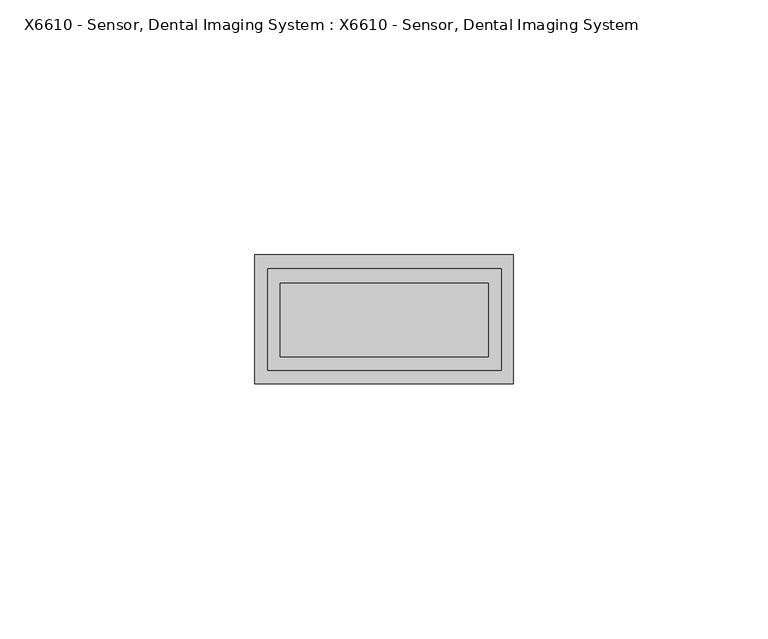
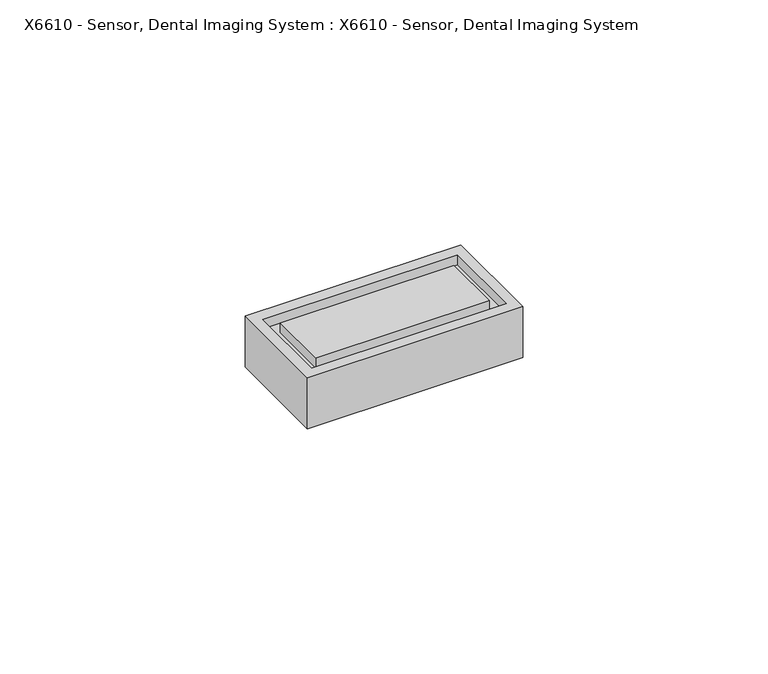
"""IFC4 building model written with IfcOpenShell, lengths in millimetres: proxy geometry, X6610 - Sensor, Dental Imaging System : X6610 - Sensor, Dental Imaging System."""

from ifc_helpers import new_model, si_unit, frame, origin, place, context, project, spatial, polyline, outline, extrude, faceted_brep, source, transform, mapped, element, save


def x6610_sensor_dental_imaging_system_x6610_sensor_dental_c57a1d08(model_context):
    return source(origin(), model_context, "Body", "SolidModel", [
        extrude(outline(polyline([(20.4811453, 7.060747), (20.4811453, -7.3741427), (-20.3347495, -7.3741427), (-20.3347495, 7.060747), (20.4811453, 7.060747)])), frame((0.0, 0.0, 10.2472794), z_axis=(0.0, 0.0, 1.0), x_axis=(1.0, 0.0, 0.0)), (0.0, 0.0, 1.0), 2.4527206),
        faceted_brep([(25.4, -12.7, 12.7), (-25.4, -12.7, 12.7), (-25.4, -12.7, 0.0), (25.4, -12.7, 0.0), (25.4, 12.7, 12.7), (25.4, 12.7, 0.0), (-25.4, 12.7, 0.0), (-25.4, 12.7, 12.7), (-22.8050147, 9.9039698, 12.7), (22.9818235, 9.9039698, 12.7), (22.9818235, -10.029614, 12.7), (-22.8050147, -10.029614, 12.7), (25.4, -5.9907412, 2.9524929), (25.4, -5.9907412, 7.2153756), (25.4, 6.0970829, 7.2153756), (25.4, 6.0970829, 2.9524929), (22.9818235, 9.9039698, 10.2472794), (-22.8050147, 9.9039698, 10.2472794), (-22.8050147, -10.029614, 10.2472794), (22.9818235, -10.029614, 10.2472794), (17.7337242, -5.9907412, 7.2153756), (17.7337242, -5.9907412, 2.9524929), (17.7337242, 6.0970829, 2.9524929), (17.7337242, 6.0970829, 7.2153756)], [[[0, 1, 2, 3]], [[4, 5, 6, 7]], [[1, 0, 4, 7], [8, 9, 10, 11]], [[2, 1, 7, 6]], [[3, 2, 6, 5]], [[0, 3, 5, 4], [12, 13, 14, 15]], [[16, 17, 18, 19]], [[17, 16, 9, 8]], [[18, 17, 8, 11]], [[19, 18, 11, 10]], [[16, 19, 10, 9]], [[20, 21, 22, 23]], [[21, 20, 13, 12]], [[22, 21, 12, 15]], [[23, 22, 15, 14]], [[20, 23, 14, 13]]]),
        faceted_brep([(-25.4, 12.7, 12.7), (-25.4, 0.0, 12.7), (-25.4, -12.7, 12.7), (25.4, -12.7, 12.7), (25.4, 12.7, 12.7), (-22.8050147, 9.9039698, 12.7), (22.9818235, 9.9039698, 12.7), (22.9818235, -10.029614, 12.7), (-22.8050147, -10.029614, 12.7), (-25.4, 12.7, 0.0), (25.4, 12.7, 0.0), (25.4, -12.7, 0.0), (-25.4, -12.7, 0.0), (-25.4, 0.0, 0.0), (25.4, -5.9907412, 2.9524929), (25.4, -5.9907412, 7.2153756), (25.4, 6.0970829, 7.2153756), (25.4, 6.0970829, 2.9524929), (22.9818235, 9.9039698, 10.2472794), (-22.8050147, 9.9039698, 10.2472794), (-22.8050147, -10.029614, 10.2472794), (22.9818235, -10.029614, 10.2472794), (17.7337242, -5.9907412, 7.2153756), (17.7337242, -5.9907412, 2.9524929), (17.7337242, 6.0970829, 2.9524929), (17.7337242, 6.0970829, 7.2153756)], [[[0, 1, 2, 3, 4], [5, 6, 7, 8]], [[9, 10, 11, 12, 13]], [[1, 0, 9, 13]], [[2, 1, 13, 12]], [[3, 2, 12, 11]], [[4, 3, 11, 10], [14, 15, 16, 17]], [[0, 4, 10, 9]], [[18, 19, 20, 21]], [[19, 18, 6, 5]], [[20, 19, 5, 8]], [[21, 20, 8, 7]], [[18, 21, 7, 6]], [[22, 23, 24, 25]], [[23, 22, 15, 14]], [[24, 23, 14, 17]], [[25, 24, 17, 16]], [[22, 25, 16, 15]]]),
    ])


if __name__ == "__main__":
    model = new_model("IFC4")
    model_context = context("Model", 3, world=origin())
    ifc_project = project(units=[si_unit("LENGTHUNIT", "METRE", prefix="MILLI")], contexts=[model_context])
    site = spatial("IfcSite", under=ifc_project)
    building = spatial("IfcBuilding", under=site)
    placement = place(None, origin())
    x6610_sensor_dental_imaging_system_x6610_sensor_dental_shape = x6610_sensor_dental_imaging_system_x6610_sensor_dental_c57a1d08(model_context)
    element("IfcBuildingElementProxy", 1, Name="X6610 - Sensor, Dental Imaging System : X6610 - Sensor, Dental Imaging System", ObjectType="X6610 - Sensor, Dental Imaging System : X6610 - Sensor, Dental Imaging System", at=placement, inside=building, context=model_context, shape_type="MappedRepresentation", body=[
        mapped(x6610_sensor_dental_imaging_system_x6610_sensor_dental_shape, transform((0.0, 0.0, 0.0), x_axis=(1.0, 0.0, 0.0), y_axis=(0.0, 1.0, 0.0), z_axis=(0.0, 0.0, 1.0))),
    ])
    save(model, "model.ifc")

# Revit data of these elements
# Type "X6610 - Sensor, Dental Imaging System : X6610 - Sensor, Dental Imaging System"
#   Watts2 = "0"
#   Watts1 = "0"
#   Unit_Issue = "EA"
#   UTIL_6_Misc = "-"
#   UTIL_5_NonMedGas = "-"
#   UTIL_4_MiscGas = "-"
#   UTIL_3_MedGas = "-"
#   UTIL_2_Elec = "-"
#   UTIL_1_WaterDrain = "-"
#   Nomenclature = "Sensor, Dental Imaging System"
#   NSN = ""
#   Location [instance default] = ""
#   JSN = "X6610"
#   Fund_Source_VA = "-"
#   Fund_Source_Navy = "-"
#   Fund_Source_Army = "-"
#   Fund_Source_AF = "-"
#   ELEC_Volts2 = "0"
#   ELEC_Volts1 = "0"
#   ELEC_Phase2 = "0"
#   ELEC_Phase1 = "0"
#   ELEC_HertzSwitch = "0"
#   ELEC_HertzDependent = "0"
#   ELEC_Hertz = "0"
#   ELEC_Amps2 = "0"
#   ELEC_Amps1 = "0"
#   DetailDescription = "A filmless digital imaging system using a sensor to acquire and digitize dental x-ray images for viewing, storing or printing. The sensor is used in conjunction with a film based x-ray system. Images are digitized and transmitted to a computer via a standard USB port and is compatible with laptop or desktop systems."
#   CAT_VA = "C"
#   CAT_Navy = "C"
#   CAT_IHS = "-"
#   CAT_Army = "C"
#   CAT_AF = "C"
#   BTUperhour = "0"
#   Weight_IP = 3
#   DIM_Width_IP = 0' - 2"
#   DIM_Height_IP = 0' - 0 1/2"
#   DIM_Depth_IP = 0' - 1"
# Element 1 (IfcBuildingElementProxy, "X6610 - Sensor, Dental Imaging System : X6610 - Sensor, Dental Imaging System")
#   Materials on its faces: "EquipSpace"
# Materials
#   "EquipSpace": class "Unassigned", colour RGB 221 217 195, transparency 0.5
